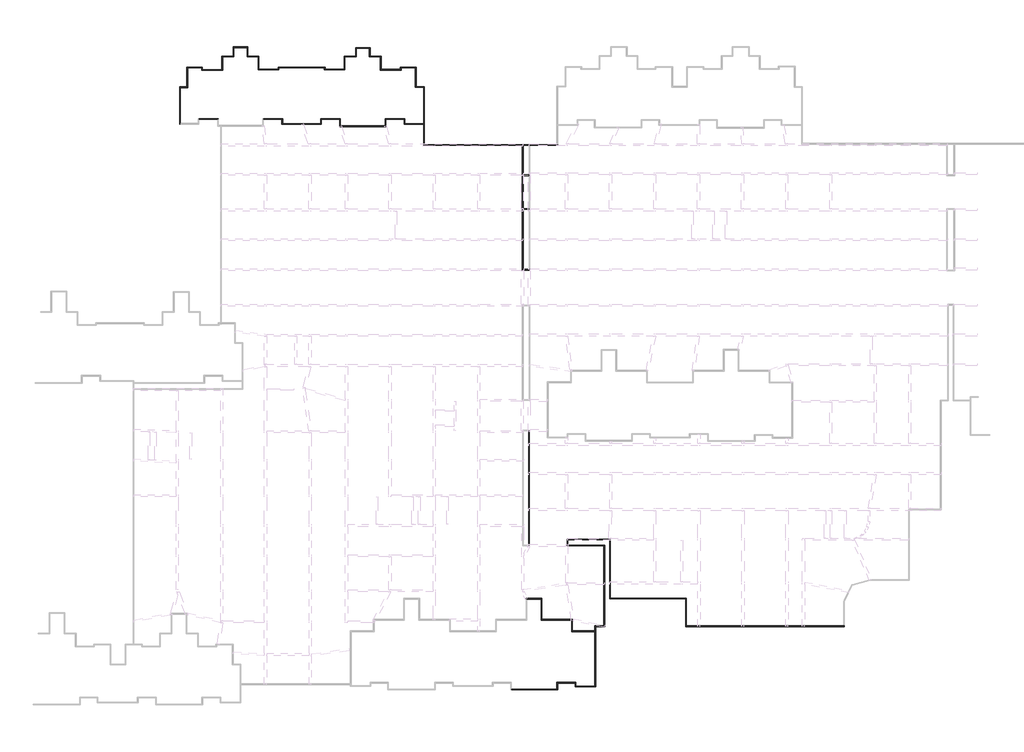
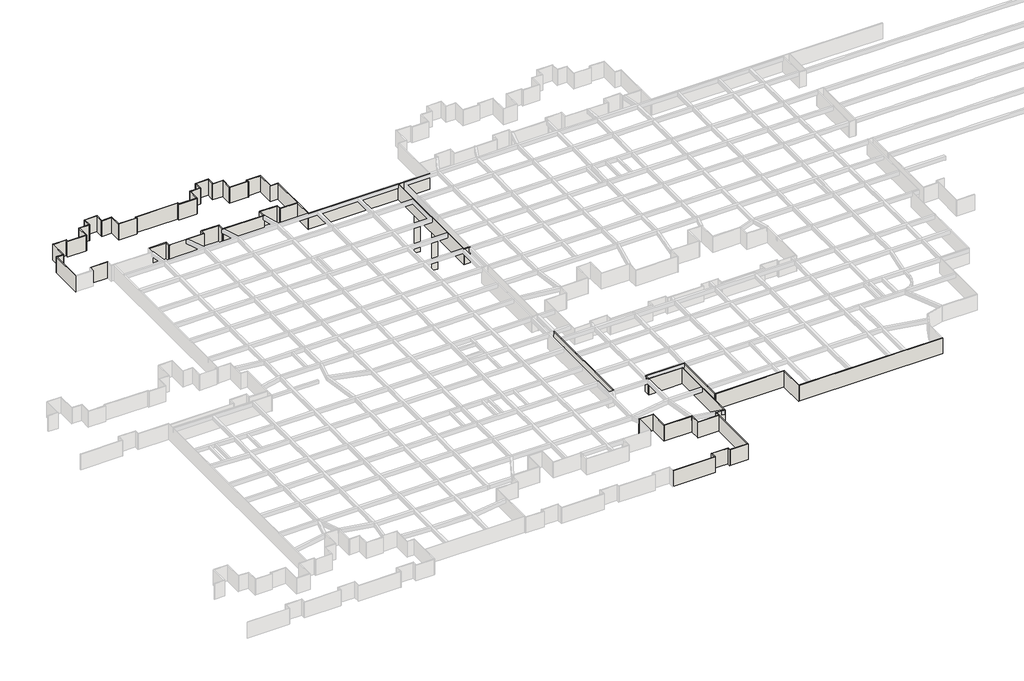
# One storey, part 3 of 16: 69 walls.
"""IFC4 building model written with IfcOpenShell, lengths in millimetres."""

from ifc_helpers import new_model, si_unit, frame, origin, origin_with_axes, place, context, project, spatial, polyline, outline, extrude, faceted_brep, element, save

model = new_model("IFC4")

# Units and contexts
model_context = context("Model", 3, world=origin())
ifc_project = project(units=[si_unit("LENGTHUNIT", "METRE", prefix="MILLI")], contexts=[model_context])

# Site, building, storey
site = spatial("IfcSite", under=ifc_project)
building = spatial("IfcBuilding", under=site)
storey = spatial("IfcBuildingStorey", under=building, Name="户型图", Elevation=0.0)

# Walls
placement = place(None, origin())
element("IfcWall", 1, ObjectType="所有墙体", at=placement, inside=storey, context=model_context, shape_type="Brep", body=[
    faceted_brep([(194060.3346415, -118367.7118415, 0.0), (194060.3346415, -121966.8447717, 0.0), (194060.3346415, -122086.8447717, 0.0), (194060.3346415, -122086.8447717, 3300.0), (194060.3346415, -121966.8447717, 3300.0), (194060.3346415, -118367.7118415, 3300.0), (194180.3346415, -118367.7118415, 0.0), (194180.3346415, -118367.7118415, 3300.0), (194180.3346415, -118487.7118415, 3300.0), (194180.3346415, -122086.8447717, 3300.0), (194180.3346415, -122086.8447717, 0.0), (194180.3346415, -118487.7118415, 0.0)], [[[0, 1, 2, 3, 4, 5]], [[6, 7, 8, 9, 10, 11]], [[2, 1, 0, 6, 11, 10]], [[5, 4, 3, 9, 8, 7]], [[3, 2, 10, 9]], [[0, 5, 7, 6]]]),
])
element("IfcWall", 2, ObjectType="所有墙体", at=placement, inside=storey, context=model_context, shape_type="Brep", body=[
    faceted_brep([(194060.3346415, -121966.8447717, 0.0), (192706.317546, -121966.8447717, 0.0), (192706.317546, -121966.8447717, 3300.0), (194060.3346415, -121966.8447717, 3300.0), (194060.3346415, -122086.8447717, 0.0), (194060.3346415, -122086.8447717, 3300.0), (192826.317546, -122086.8447717, 3300.0), (192706.317546, -122086.8447717, 3300.0), (192706.317546, -122086.8447717, 0.0), (192826.317546, -122086.8447717, 0.0)], [[[0, 1, 2, 3]], [[4, 5, 6, 7, 8, 9]], [[1, 0, 4, 9, 8]], [[3, 2, 7, 6, 5]], [[0, 3, 5, 4]], [[2, 1, 8, 7]]]),
])
element("IfcWall", 3, ObjectType="所有墙体", at=placement, inside=storey, context=model_context, shape_type="Brep", body=[
    faceted_brep([(192706.317546, -122086.8447717, 0.0), (192706.317546, -128736.151487, 0.0), (192706.317546, -128736.151487, 3300.0), (192706.317546, -122086.8447717, 3300.0), (192826.317546, -122086.8447717, 0.0), (192826.317546, -122086.8447717, 3300.0), (192826.317546, -128616.151487, 3300.0), (192826.317546, -128736.151487, 3300.0), (192826.317546, -128736.151487, 0.0), (192826.317546, -128616.151487, 0.0)], [[[0, 1, 2, 3]], [[4, 5, 6, 7, 8, 9]], [[1, 0, 4, 9, 8]], [[3, 2, 7, 6, 5]], [[0, 3, 5, 4]], [[2, 1, 8, 7]]]),
])
element("IfcWall", 4, ObjectType="所有墙体", at=placement, inside=storey, context=model_context, shape_type="Brep", body=[
    faceted_brep([(196226.317546, -127836.151487, 0.0), (199599.9062186, -127836.151487, 0.0), (199719.9062186, -127836.151487, 0.0), (199719.9062186, -127836.151487, 3300.0), (199599.9062186, -127836.151487, 3300.0), (196226.317546, -127836.151487, 3300.0), (196226.317546, -127716.151487, 0.0), (196226.317546, -127716.151487, 3300.0), (199719.9062186, -127716.151487, 3300.0), (199719.9062186, -127716.151487, 0.0)], [[[0, 1, 2, 3, 4, 5]], [[6, 7, 8, 9]], [[2, 1, 0, 6, 9]], [[5, 4, 3, 8, 7]], [[0, 5, 7, 6]], [[3, 2, 9, 8]]]),
])
element("IfcWall", 5, ObjectType="所有墙体", at=placement, inside=storey, context=model_context, shape_type="Brep", body=[
    faceted_brep([(207918.5069416, -127836.151487, 0.0), (211299.9135032, -127836.151487, 0.0), (211419.9135032, -127836.151487, 0.0), (211419.9135032, -127836.151487, 3300.0), (211299.9135032, -127836.151487, 3300.0), (207918.5069416, -127836.151487, 3300.0), (207918.5069416, -127716.151487, 0.0), (207918.5069416, -127716.151487, 3300.0), (211419.9135032, -127716.151487, 3300.0), (211419.9135032, -127716.151487, 0.0)], [[[0, 1, 2, 3, 4, 5]], [[6, 7, 8, 9]], [[2, 1, 0, 6, 9]], [[5, 4, 3, 8, 7]], [[0, 5, 7, 6]], [[3, 2, 9, 8]]]),
])
element("IfcWall", 6, ObjectType="所有墙体", at=placement, inside=storey, context=model_context, shape_type="Brep", body=[
    faceted_brep([(211299.9135032, -127836.151487, 0.0), (211299.9135032, -128756.8999905, 0.0), (211299.9135032, -128756.8999905, 3300.0), (211299.9135032, -127836.151487, 3300.0), (211419.9135032, -127836.151487, 0.0), (211419.9135032, -127836.151487, 3300.0), (211419.9135032, -128636.8999905, 3300.0), (211419.9135032, -128756.8999905, 3300.0), (211419.9135032, -128756.8999905, 0.0), (211419.9135032, -128636.8999905, 0.0)], [[[0, 1, 2, 3]], [[4, 5, 6, 7, 8, 9]], [[1, 0, 4, 9, 8]], [[3, 2, 7, 6, 5]], [[0, 3, 5, 4]], [[2, 1, 8, 7]]]),
])
element("IfcWall", 7, ObjectType="所有墙体", at=placement, inside=storey, context=model_context, shape_type="Brep", body=[
    faceted_brep([(211419.9135032, -128756.8999905, 0.0), (218418.8904026, -128756.8999905, 0.0), (218418.8904026, -128756.8999905, 3300.0), (211419.9135032, -128756.8999905, 3300.0), (211419.9135032, -128636.8999905, 0.0), (211419.9135032, -128636.8999905, 3300.0), (218298.8904026, -128636.8999905, 3300.0), (218418.8904026, -128636.8999905, 3300.0), (218418.8904026, -128636.8999905, 0.0), (218298.8904026, -128636.8999905, 0.0)], [[[0, 1, 2, 3]], [[4, 5, 6, 7, 8, 9]], [[1, 0, 4, 9, 8]], [[3, 2, 7, 6, 5]], [[0, 3, 5, 4]], [[2, 1, 8, 7]]]),
])
element("IfcWall", 8, ObjectType="所有墙体", at=placement, inside=storey, context=model_context, shape_type="Brep", body=[
    faceted_brep([(218418.8904026, -128636.8999905, 0.0), (218418.8904026, -127836.151487, 0.0), (218418.8904026, -127716.151487, 0.0), (218418.8904026, -127716.151487, 3300.0), (218418.8904026, -127836.151487, 3300.0), (218418.8904026, -128636.8999905, 3300.0), (218298.8904026, -128636.8999905, 0.0), (218298.8904026, -128636.8999905, 3300.0), (218298.8904026, -127716.151487, 3300.0), (218298.8904026, -127716.151487, 0.0)], [[[0, 1, 2, 3, 4, 5]], [[6, 7, 8, 9]], [[2, 1, 0, 6, 9]], [[5, 4, 3, 8, 7]], [[0, 5, 7, 6]], [[3, 2, 9, 8]]]),
])
element("IfcWall", 9, ObjectType="所有墙体", at=placement, inside=storey, context=model_context, shape_type="Brep", body=[
    faceted_brep([(218418.8904026, -127836.151487, 0.0), (221799.9200406, -127836.151487, 0.0), (221919.9200406, -127836.151487, 0.0), (221919.9200406, -127836.151487, 3300.0), (221799.9200406, -127836.151487, 3300.0), (218418.8904026, -127836.151487, 3300.0), (218418.8904026, -127716.151487, 0.0), (218418.8904026, -127716.151487, 3300.0), (221919.9200406, -127716.151487, 3300.0), (221919.9200406, -127716.151487, 0.0)], [[[0, 1, 2, 3, 4, 5]], [[6, 7, 8, 9]], [[2, 1, 0, 6, 9]], [[5, 4, 3, 8, 7]], [[0, 5, 7, 6]], [[3, 2, 9, 8]]]),
])
element("IfcWall", 10, ObjectType="所有墙体", at=placement, inside=storey, context=model_context, shape_type="Brep", body=[
    faceted_brep([(221799.9200406, -127836.151487, 0.0), (221799.9200406, -129168.6171458, 0.0), (221799.9200406, -129168.6171458, 3300.0), (221799.9200406, -127836.151487, 3300.0), (221919.9200406, -127836.151487, 0.0), (221919.9200406, -127836.151487, 3300.0), (221919.9200406, -129048.6171458, 3300.0), (221919.9200406, -129168.6171458, 3300.0), (221919.9200406, -129168.6171458, 0.0), (221919.9200406, -129048.6171458, 0.0)], [[[0, 1, 2, 3]], [[4, 5, 6, 7, 8, 9]], [[1, 0, 4, 9, 8]], [[3, 2, 7, 6, 5]], [[0, 3, 5, 4]], [[2, 1, 8, 7]]]),
])
element("IfcWall", 11, ObjectType="所有墙体", at=placement, inside=storey, context=model_context, shape_type="Brep", body=[
    faceted_brep([(221919.9200406, -129168.6171458, 0.0), (230118.438254, -129168.6171458, 0.0), (230118.438254, -129168.6171458, 3300.0), (221919.9200406, -129168.6171458, 3300.0), (221919.9200406, -129048.6171458, 0.0), (221919.9200406, -129048.6171458, 3300.0), (229998.438254, -129048.6171458, 3300.0), (230118.438254, -129048.6171458, 3300.0), (230118.438254, -129048.6171458, 0.0), (229998.438254, -129048.6171458, 0.0)], [[[0, 1, 2, 3]], [[4, 5, 6, 7, 8, 9]], [[1, 0, 4, 9, 8]], [[3, 2, 7, 6, 5]], [[0, 3, 5, 4]], [[2, 1, 8, 7]]]),
])
element("IfcWall", 12, ObjectType="所有墙体", at=placement, inside=storey, context=model_context, shape_type="Brep", body=[
    faceted_brep([(230118.438254, -129048.6171458, 0.0), (230118.438254, -127836.151487, 0.0), (230118.438254, -127716.151487, 0.0), (230118.438254, -127716.151487, 3300.0), (230118.438254, -127836.151487, 3300.0), (230118.438254, -129048.6171458, 3300.0), (229998.438254, -129048.6171458, 0.0), (229998.438254, -129048.6171458, 3300.0), (229998.438254, -127716.151487, 3300.0), (229998.438254, -127716.151487, 0.0)], [[[0, 1, 2, 3, 4, 5]], [[6, 7, 8, 9]], [[2, 1, 0, 6, 9]], [[5, 4, 3, 8, 7]], [[0, 5, 7, 6]], [[3, 2, 9, 8]]]),
])
element("IfcWall", 13, ObjectType="所有墙体", at=placement, inside=storey, context=model_context, shape_type="Brep", body=[
    faceted_brep([(230118.438254, -127836.151487, 0.0), (233499.9273251, -127836.151487, 0.0), (233619.9273251, -127836.151487, 0.0), (233619.9273251, -127836.151487, 3300.0), (233499.9273251, -127836.151487, 3300.0), (230118.438254, -127836.151487, 3300.0), (230118.438254, -127716.151487, 0.0), (230118.438254, -127716.151487, 3300.0), (233619.9273251, -127716.151487, 3300.0), (233619.9273251, -127716.151487, 0.0)], [[[0, 1, 2, 3, 4, 5]], [[6, 7, 8, 9]], [[2, 1, 0, 6, 9]], [[5, 4, 3, 8, 7]], [[0, 5, 7, 6]], [[3, 2, 9, 8]]]),
])
element("IfcWall", 14, ObjectType="所有墙体", at=placement, inside=storey, context=model_context, shape_type="Brep", body=[
    faceted_brep([(233499.9273251, -127836.151487, 0.0), (233499.9273251, -128756.8999905, 0.0), (233499.9273251, -128756.8999905, 3300.0), (233499.9273251, -127836.151487, 3300.0), (233619.9273251, -127836.151487, 0.0), (233619.9273251, -127836.151487, 3300.0), (233619.9273251, -128636.8999905, 3300.0), (233619.9273251, -128756.8999905, 3300.0), (233619.9273251, -128756.8999905, 0.0), (233619.9273251, -128636.8999905, 0.0)], [[[0, 1, 2, 3]], [[4, 5, 6, 7, 8, 9]], [[1, 0, 4, 9, 8]], [[3, 2, 7, 6, 5]], [[0, 3, 5, 4]], [[2, 1, 8, 7]]]),
])
element("IfcWall", 15, ObjectType="所有墙体", at=placement, inside=storey, context=model_context, shape_type="SweptSolid", body=[
    extrude(outline(polyline([(237002.7517568, -128756.8999905), (233619.9273251, -128756.8999905), (233619.9273251, -128636.8999905), (237002.7517568, -128636.8999905), (237002.7517568, -128756.8999905)])), origin_with_axes(), (0.0, 0.0, 1.0), 3300.0),
])
element("IfcWall", 16, ObjectType="所有墙体", at=placement, inside=storey, context=model_context, shape_type="Brep", body=[
    faceted_brep([(237122.7517568, -132556.8999905, 0.0), (237122.7517568, -132436.8999905, 0.0), (237122.7517568, -121914.0192789, 0.0), (237122.7517568, -121914.0192789, 3300.0), (237122.7517568, -132436.8999905, 3300.0), (237122.7517568, -132556.8999905, 3300.0), (237002.7517568, -132556.8999905, 0.0), (237002.7517568, -132556.8999905, 3300.0), (237002.7517568, -128756.8999905, 3300.0), (237002.7517568, -128636.8999905, 3300.0), (237002.7517568, -122034.0192789, 3300.0), (237002.7517568, -121914.0192789, 3300.0), (237002.7517568, -121914.0192789, 0.0), (237002.7517568, -122034.0192789, 0.0), (237002.7517568, -128636.8999905, 0.0), (237002.7517568, -128756.8999905, 0.0)], [[[0, 1, 2, 3, 4, 5]], [[6, 7, 8, 9, 10, 11, 12, 13, 14, 15]], [[2, 1, 0, 6, 15, 14, 13, 12]], [[5, 4, 3, 11, 10, 9, 8, 7]], [[3, 2, 12, 11]], [[0, 5, 7, 6]]]),
])
element("IfcWall", 17, ObjectType="所有墙体", at=placement, inside=storey, context=model_context, shape_type="Brep", body=[
    faceted_brep([(237002.7517568, -121914.0192789, 0.0), (235628.9140291, -121914.0192789, 0.0), (235508.9140291, -121914.0192789, 0.0), (235508.9140291, -121914.0192789, 3300.0), (235628.9140291, -121914.0192789, 3300.0), (237002.7517568, -121914.0192789, 3300.0), (237002.7517568, -122034.0192789, 0.0), (237002.7517568, -122034.0192789, 3300.0), (235508.9140291, -122034.0192789, 3300.0), (235508.9140291, -122034.0192789, 0.0)], [[[0, 1, 2, 3, 4, 5]], [[6, 7, 8, 9]], [[2, 1, 0, 6, 9]], [[5, 4, 3, 8, 7]], [[0, 5, 7, 6]], [[3, 2, 9, 8]]]),
])
element("IfcWall", 18, ObjectType="所有墙体", at=placement, inside=storey, context=model_context, shape_type="Brep", body=[
    faceted_brep([(235628.9140291, -121914.0192789, 0.0), (235628.9140291, -118412.2081323, 0.0), (235628.9140291, -118412.2081323, 3300.0), (235628.9140291, -121914.0192789, 3300.0), (235508.9140291, -121914.0192789, 0.0), (235508.9140291, -121914.0192789, 3300.0), (235508.9140291, -118532.2081323, 3300.0), (235508.9140291, -118412.2081323, 3300.0), (235508.9140291, -118412.2081323, 0.0), (235508.9140291, -118532.2081323, 0.0)], [[[0, 1, 2, 3]], [[4, 5, 6, 7, 8, 9]], [[1, 0, 4, 9, 8]], [[3, 2, 7, 6, 5]], [[0, 3, 5, 4]], [[2, 1, 8, 7]]]),
])
element("IfcWall", 19, ObjectType="所有墙体", at=placement, inside=storey, context=model_context, shape_type="Brep", body=[
    faceted_brep([(235508.9140291, -118412.2081323, 0.0), (232809.8642198, -118412.2081323, 0.0), (232809.8642198, -118412.2081323, 3300.0), (235508.9140291, -118412.2081323, 3300.0), (235508.9140291, -118532.2081323, 0.0), (235508.9140291, -118532.2081323, 3300.0), (232929.8642198, -118532.2081323, 3300.0), (232809.8642198, -118532.2081323, 3300.0), (232809.8642198, -118532.2081323, 0.0), (232929.8642198, -118532.2081323, 0.0)], [[[0, 1, 2, 3]], [[4, 5, 6, 7, 8, 9]], [[1, 0, 4, 9, 8]], [[3, 2, 7, 6, 5]], [[0, 3, 5, 4]], [[2, 1, 8, 7]]]),
])
element("IfcWall", 20, ObjectType="所有墙体", at=placement, inside=storey, context=model_context, shape_type="Brep", body=[
    faceted_brep([(232809.8642198, -118532.2081323, 0.0), (232809.8642198, -118808.218552, 0.0), (232809.8642198, -118928.218552, 0.0), (232809.8642198, -118928.218552, 3300.0), (232809.8642198, -118808.218552, 3300.0), (232809.8642198, -118532.2081323, 3300.0), (232929.8642198, -118532.2081323, 0.0), (232929.8642198, -118532.2081323, 3300.0), (232929.8642198, -118928.218552, 3300.0), (232929.8642198, -118928.218552, 0.0)], [[[0, 1, 2, 3, 4, 5]], [[6, 7, 8, 9]], [[2, 1, 0, 6, 9]], [[5, 4, 3, 8, 7]], [[0, 5, 7, 6]], [[3, 2, 9, 8]]]),
])
element("IfcWall", 21, ObjectType="所有墙体", at=placement, inside=storey, context=model_context, shape_type="Brep", body=[
    faceted_brep([(232809.8642198, -118808.218552, 0.0), (229282.488847, -118808.218552, 0.0), (229162.488847, -118808.218552, 0.0), (229162.488847, -118808.218552, 3300.0), (229282.488847, -118808.218552, 3300.0), (232809.8642198, -118808.218552, 3300.0), (232809.8642198, -118928.218552, 0.0), (232809.8642198, -118928.218552, 3300.0), (229162.488847, -118928.218552, 3300.0), (229162.488847, -118928.218552, 0.0)], [[[0, 1, 2, 3, 4, 5]], [[6, 7, 8, 9]], [[2, 1, 0, 6, 9]], [[5, 4, 3, 8, 7]], [[0, 5, 7, 6]], [[3, 2, 9, 8]]]),
])
element("IfcWall", 22, ObjectType="所有墙体", at=placement, inside=storey, context=model_context, shape_type="Brep", body=[
    faceted_brep([(229282.488847, -118808.218552, 0.0), (229282.488847, -116405.5418968, 0.0), (229282.488847, -116405.5418968, 3300.0), (229282.488847, -118808.218552, 3300.0), (229162.488847, -118808.218552, 0.0), (229162.488847, -118808.218552, 3300.0), (229162.488847, -116525.5418968, 3300.0), (229162.488847, -116405.5418968, 3300.0), (229162.488847, -116405.5418968, 0.0), (229162.488847, -116525.5418968, 0.0)], [[[0, 1, 2, 3]], [[4, 5, 6, 7, 8, 9]], [[1, 0, 4, 9, 8]], [[3, 2, 7, 6, 5]], [[0, 3, 5, 4]], [[2, 1, 8, 7]]]),
])
element("IfcWall", 23, ObjectType="所有墙体", at=placement, inside=storey, context=model_context, shape_type="Brep", body=[
    faceted_brep([(229162.488847, -116405.5418968, 0.0), (227283.5491439, -116405.5418968, 0.0), (227163.5491439, -116405.5418968, 0.0), (227163.5491439, -116405.5418968, 3300.0), (227283.5491439, -116405.5418968, 3300.0), (229162.488847, -116405.5418968, 3300.0), (229162.488847, -116525.5418968, 0.0), (229162.488847, -116525.5418968, 3300.0), (227163.5491439, -116525.5418968, 3300.0), (227163.5491439, -116525.5418968, 0.0)], [[[0, 1, 2, 3, 4, 5]], [[6, 7, 8, 9]], [[2, 1, 0, 6, 9]], [[5, 4, 3, 8, 7]], [[0, 5, 7, 6]], [[3, 2, 9, 8]]]),
])
element("IfcWall", 24, ObjectType="所有墙体", at=placement, inside=storey, context=model_context, shape_type="Brep", body=[
    faceted_brep([(227283.5491439, -116405.5418968, 0.0), (227283.5491439, -114851.8046012, 0.0), (227283.5491439, -114851.8046012, 3300.0), (227283.5491439, -116405.5418968, 3300.0), (227163.5491439, -116405.5418968, 0.0), (227163.5491439, -116405.5418968, 3300.0), (227163.5491439, -114971.8046012, 3300.0), (227163.5491439, -114851.8046012, 3300.0), (227163.5491439, -114851.8046012, 0.0), (227163.5491439, -114971.8046012, 0.0)], [[[0, 1, 2, 3]], [[4, 5, 6, 7, 8, 9]], [[1, 0, 4, 9, 8]], [[3, 2, 7, 6, 5]], [[0, 3, 5, 4]], [[2, 1, 8, 7]]]),
])
element("IfcWall", 25, ObjectType="所有墙体", at=placement, inside=storey, context=model_context, shape_type="Brep", body=[
    faceted_brep([(227163.5491439, -114851.8046012, 0.0), (224663.3843746, -114851.8046012, 0.0), (224663.3843746, -114851.8046012, 3300.0), (227163.5491439, -114851.8046012, 3300.0), (227163.5491439, -114971.8046012, 0.0), (227163.5491439, -114971.8046012, 3300.0), (224783.3843746, -114971.8046012, 3300.0), (224663.3843746, -114971.8046012, 3300.0), (224663.3843746, -114971.8046012, 0.0), (224783.3843746, -114971.8046012, 0.0)], [[[0, 1, 2, 3]], [[4, 5, 6, 7, 8, 9]], [[1, 0, 4, 9, 8]], [[3, 2, 7, 6, 5]], [[0, 3, 5, 4]], [[2, 1, 8, 7]]]),
])
element("IfcWall", 26, ObjectType="所有墙体", at=placement, inside=storey, context=model_context, shape_type="Brep", body=[
    faceted_brep([(224663.3843746, -114971.8046012, 0.0), (224663.3843746, -116405.5418968, 0.0), (224663.3843746, -116525.5418968, 0.0), (224663.3843746, -116525.5418968, 3300.0), (224663.3843746, -116405.5418968, 3300.0), (224663.3843746, -114971.8046012, 3300.0), (224783.3843746, -114971.8046012, 0.0), (224783.3843746, -114971.8046012, 3300.0), (224783.3843746, -116525.5418968, 3300.0), (224783.3843746, -116525.5418968, 0.0)], [[[0, 1, 2, 3, 4, 5]], [[6, 7, 8, 9]], [[2, 1, 0, 6, 9]], [[5, 4, 3, 8, 7]], [[0, 5, 7, 6]], [[3, 2, 9, 8]]]),
])
element("IfcWall", 27, ObjectType="所有墙体", at=placement, inside=storey, context=model_context, shape_type="Brep", body=[
    faceted_brep([(224663.3843746, -116405.5418968, 0.0), (222610.0704279, -116405.5418968, 0.0), (222610.0704279, -116405.5418968, 3300.0), (224663.3843746, -116405.5418968, 3300.0), (224663.3843746, -116525.5418968, 0.0), (224663.3843746, -116525.5418968, 3300.0), (222730.0704279, -116525.5418968, 3300.0), (222610.0704279, -116525.5418968, 3300.0), (222610.0704279, -116525.5418968, 0.0), (222730.0704279, -116525.5418968, 0.0)], [[[0, 1, 2, 3]], [[4, 5, 6, 7, 8, 9]], [[1, 0, 4, 9, 8]], [[3, 2, 7, 6, 5]], [[0, 3, 5, 4]], [[2, 1, 8, 7]]]),
])
element("IfcWall", 28, ObjectType="所有墙体", at=placement, inside=storey, context=model_context, shape_type="Brep", body=[
    faceted_brep([(222610.0704279, -116525.5418968, 0.0), (222610.0704279, -118749.3864331, 0.0), (222610.0704279, -118869.3864331, 0.0), (222610.0704279, -118869.3864331, 3300.0), (222610.0704279, -118749.3864331, 3300.0), (222610.0704279, -116525.5418968, 3300.0), (222730.0704279, -116525.5418968, 0.0), (222730.0704279, -116525.5418968, 3300.0), (222730.0704279, -118869.3864331, 3300.0), (222730.0704279, -118869.3864331, 0.0)], [[[0, 1, 2, 3, 4, 5]], [[6, 7, 8, 9]], [[2, 1, 0, 6, 9]], [[5, 4, 3, 8, 7]], [[0, 5, 7, 6]], [[3, 2, 9, 8]]]),
])
element("IfcWall", 29, ObjectType="所有墙体", at=placement, inside=storey, context=model_context, shape_type="Brep", body=[
    faceted_brep([(222610.0704279, -118749.3864331, 0.0), (219130.3191805, -118749.3864331, 0.0), (219010.3191805, -118749.3864331, 0.0), (219010.3191805, -118749.3864331, 3300.0), (219130.3191805, -118749.3864331, 3300.0), (222610.0704279, -118749.3864331, 3300.0), (222610.0704279, -118869.3864331, 0.0), (222610.0704279, -118869.3864331, 3300.0), (219010.3191805, -118869.3864331, 3300.0), (219010.3191805, -118869.3864331, 0.0)], [[[0, 1, 2, 3, 4, 5]], [[6, 7, 8, 9]], [[2, 1, 0, 6, 9]], [[5, 4, 3, 8, 7]], [[0, 5, 7, 6]], [[3, 2, 9, 8]]]),
])
element("IfcWall", 30, ObjectType="所有墙体", at=placement, inside=storey, context=model_context, shape_type="Brep", body=[
    faceted_brep([(219130.3191805, -118749.3864331, 0.0), (219130.3191805, -118390.5039842, 0.0), (219130.3191805, -118390.5039842, 3300.0), (219130.3191805, -118749.3864331, 3300.0), (219010.3191805, -118749.3864331, 0.0), (219010.3191805, -118749.3864331, 3300.0), (219010.3191805, -118510.5039842, 3300.0), (219010.3191805, -118390.5039842, 3300.0), (219010.3191805, -118390.5039842, 0.0), (219010.3191805, -118510.5039842, 0.0)], [[[0, 1, 2, 3]], [[4, 5, 6, 7, 8, 9]], [[1, 0, 4, 9, 8]], [[3, 2, 7, 6, 5]], [[0, 3, 5, 4]], [[2, 1, 8, 7]]]),
])
element("IfcWall", 31, ObjectType="所有墙体", at=placement, inside=storey, context=model_context, shape_type="Brep", body=[
    faceted_brep([(219010.3191805, -118390.5039842, 0.0), (210609.9338471, -118390.5039842, 0.0), (210609.9338471, -118390.5039842, 3300.0), (219010.3191805, -118390.5039842, 3300.0), (219010.3191805, -118510.5039842, 0.0), (219010.3191805, -118510.5039842, 3300.0), (210729.9338471, -118510.5039842, 3300.0), (210609.9338471, -118510.5039842, 3300.0), (210609.9338471, -118510.5039842, 0.0), (210729.9338471, -118510.5039842, 0.0)], [[[0, 1, 2, 3]], [[4, 5, 6, 7, 8, 9]], [[1, 0, 4, 9, 8]], [[3, 2, 7, 6, 5]], [[0, 3, 5, 4]], [[2, 1, 8, 7]]]),
])
element("IfcWall", 32, ObjectType="所有墙体", at=placement, inside=storey, context=model_context, shape_type="Brep", body=[
    faceted_brep([(210609.9338471, -118510.5039842, 0.0), (210609.9338471, -118749.3864331, 0.0), (210609.9338471, -118869.3864331, 0.0), (210609.9338471, -118869.3864331, 3300.0), (210609.9338471, -118749.3864331, 3300.0), (210609.9338471, -118510.5039842, 3300.0), (210729.9338471, -118510.5039842, 0.0), (210729.9338471, -118510.5039842, 3300.0), (210729.9338471, -118869.3864331, 3300.0), (210729.9338471, -118869.3864331, 0.0)], [[[0, 1, 2, 3, 4, 5]], [[6, 7, 8, 9]], [[2, 1, 0, 6, 9]], [[5, 4, 3, 8, 7]], [[0, 5, 7, 6]], [[3, 2, 9, 8]]]),
])
element("IfcWall", 33, ObjectType="所有墙体", at=placement, inside=storey, context=model_context, shape_type="Brep", body=[
    faceted_brep([(210609.9338471, -118749.3864331, 0.0), (207082.5026691, -118749.3864331, 0.0), (206962.5026691, -118749.3864331, 0.0), (206962.5026691, -118749.3864331, 3300.0), (207082.5026691, -118749.3864331, 3300.0), (210609.9338471, -118749.3864331, 3300.0), (210609.9338471, -118869.3864331, 0.0), (210609.9338471, -118869.3864331, 3300.0), (206962.5026691, -118869.3864331, 3300.0), (206962.5026691, -118869.3864331, 0.0)], [[[0, 1, 2, 3, 4, 5]], [[6, 7, 8, 9]], [[2, 1, 0, 6, 9]], [[5, 4, 3, 8, 7]], [[0, 5, 7, 6]], [[3, 2, 9, 8]]]),
])
element("IfcWall", 34, ObjectType="所有墙体", at=placement, inside=storey, context=model_context, shape_type="Brep", body=[
    faceted_brep([(207082.5026691, -118749.3864331, 0.0), (207082.5026691, -116405.5418968, 0.0), (207082.5026691, -116405.5418968, 3300.0), (207082.5026691, -118749.3864331, 3300.0), (206962.5026691, -118749.3864331, 0.0), (206962.5026691, -118749.3864331, 3300.0), (206962.5026691, -116525.5418968, 3300.0), (206962.5026691, -116405.5418968, 3300.0), (206962.5026691, -116405.5418968, 0.0), (206962.5026691, -116525.5418968, 0.0)], [[[0, 1, 2, 3]], [[4, 5, 6, 7, 8, 9]], [[1, 0, 4, 9, 8]], [[3, 2, 7, 6, 5]], [[0, 3, 5, 4]], [[2, 1, 8, 7]]]),
])
element("IfcWall", 35, ObjectType="所有墙体", at=placement, inside=storey, context=model_context, shape_type="Brep", body=[
    faceted_brep([(206962.5026691, -116405.5418968, 0.0), (205085.2649614, -116405.5418968, 0.0), (204965.2649614, -116405.5418968, 0.0), (204965.2649614, -116405.5418968, 3300.0), (205085.2649614, -116405.5418968, 3300.0), (206962.5026691, -116405.5418968, 3300.0), (206962.5026691, -116525.5418968, 0.0), (206962.5026691, -116525.5418968, 3300.0), (204965.2649614, -116525.5418968, 3300.0), (204965.2649614, -116525.5418968, 0.0)], [[[0, 1, 2, 3, 4, 5]], [[6, 7, 8, 9]], [[2, 1, 0, 6, 9]], [[5, 4, 3, 8, 7]], [[0, 5, 7, 6]], [[3, 2, 9, 8]]]),
])
element("IfcWall", 36, ObjectType="所有墙体", at=placement, inside=storey, context=model_context, shape_type="Brep", body=[
    faceted_brep([(205085.2649614, -116405.5418968, 0.0), (205085.2649614, -114728.4266647, 0.0), (205085.2649614, -114728.4266647, 3300.0), (205085.2649614, -116405.5418968, 3300.0), (204965.2649614, -116405.5418968, 0.0), (204965.2649614, -116405.5418968, 3300.0), (204965.2649614, -114848.4266647, 3300.0), (204965.2649614, -114728.4266647, 3300.0), (204965.2649614, -114728.4266647, 0.0), (204965.2649614, -114848.4266647, 0.0)], [[[0, 1, 2, 3]], [[4, 5, 6, 7, 8, 9]], [[1, 0, 4, 9, 8]], [[3, 2, 7, 6, 5]], [[0, 3, 5, 4]], [[2, 1, 8, 7]]]),
])
element("IfcWall", 37, ObjectType="所有墙体", at=placement, inside=storey, context=model_context, shape_type="Brep", body=[
    faceted_brep([(204965.2649614, -114728.4266647, 0.0), (202463.5082295, -114728.4266647, 0.0), (202463.5082295, -114728.4266647, 3300.0), (204965.2649614, -114728.4266647, 3300.0), (204965.2649614, -114848.4266647, 0.0), (204965.2649614, -114848.4266647, 3300.0), (202583.5082295, -114848.4266647, 3300.0), (202463.5082295, -114848.4266647, 3300.0), (202463.5082295, -114848.4266647, 0.0), (202583.5082295, -114848.4266647, 0.0)], [[[0, 1, 2, 3]], [[4, 5, 6, 7, 8, 9]], [[1, 0, 4, 9, 8]], [[3, 2, 7, 6, 5]], [[0, 3, 5, 4]], [[2, 1, 8, 7]]]),
])
element("IfcWall", 38, ObjectType="所有墙体", at=placement, inside=storey, context=model_context, shape_type="Brep", body=[
    faceted_brep([(202463.5082295, -114848.4266647, 0.0), (202463.5082295, -116405.5418968, 0.0), (202463.5082295, -116525.5418968, 0.0), (202463.5082295, -116525.5418968, 3300.0), (202463.5082295, -116405.5418968, 3300.0), (202463.5082295, -114848.4266647, 3300.0), (202583.5082295, -114848.4266647, 0.0), (202583.5082295, -114848.4266647, 3300.0), (202583.5082295, -116525.5418968, 3300.0), (202583.5082295, -116525.5418968, 0.0)], [[[0, 1, 2, 3, 4, 5]], [[6, 7, 8, 9]], [[2, 1, 0, 6, 9]], [[5, 4, 3, 8, 7]], [[0, 5, 7, 6]], [[3, 2, 9, 8]]]),
])
element("IfcWall", 39, ObjectType="所有墙体", at=placement, inside=storey, context=model_context, shape_type="Brep", body=[
    faceted_brep([(202463.5082295, -116405.5418968, 0.0), (200410.4144423, -116405.5418968, 0.0), (200410.4144423, -116405.5418968, 3300.0), (202463.5082295, -116405.5418968, 3300.0), (202463.5082295, -116525.5418968, 0.0), (202463.5082295, -116525.5418968, 3300.0), (200530.4144423, -116525.5418968, 3300.0), (200410.4144423, -116525.5418968, 3300.0), (200410.4144423, -116525.5418968, 0.0), (200530.4144423, -116525.5418968, 0.0)], [[[0, 1, 2, 3]], [[4, 5, 6, 7, 8, 9]], [[1, 0, 4, 9, 8]], [[3, 2, 7, 6, 5]], [[0, 3, 5, 4]], [[2, 1, 8, 7]]]),
])
element("IfcWall", 40, ObjectType="所有墙体", at=placement, inside=storey, context=model_context, shape_type="Brep", body=[
    faceted_brep([(200410.4144423, -116525.5418968, 0.0), (200410.4144423, -118820.6686813, 0.0), (200410.4144423, -118940.6686813, 0.0), (200410.4144423, -118940.6686813, 3300.0), (200410.4144423, -118820.6686813, 3300.0), (200410.4144423, -116525.5418968, 3300.0), (200530.4144423, -116525.5418968, 0.0), (200530.4144423, -116525.5418968, 3300.0), (200530.4144423, -118940.6686813, 3300.0), (200530.4144423, -118940.6686813, 0.0)], [[[0, 1, 2, 3, 4, 5]], [[6, 7, 8, 9]], [[2, 1, 0, 6, 9]], [[5, 4, 3, 8, 7]], [[0, 5, 7, 6]], [[3, 2, 9, 8]]]),
])
element("IfcWall", 41, ObjectType="所有墙体", at=placement, inside=storey, context=model_context, shape_type="Brep", body=[
    faceted_brep([(200410.4144423, -118820.6686813, 0.0), (196830.4144423, -118820.6686813, 0.0), (196710.4144423, -118820.6686813, 0.0), (196710.4144423, -118820.6686813, 3300.0), (196830.4144423, -118820.6686813, 3300.0), (200410.4144423, -118820.6686813, 3300.0), (200410.4144423, -118940.6686813, 0.0), (200410.4144423, -118940.6686813, 3300.0), (196710.4144423, -118940.6686813, 3300.0), (196710.4144423, -118940.6686813, 0.0)], [[[0, 1, 2, 3, 4, 5]], [[6, 7, 8, 9]], [[2, 1, 0, 6, 9]], [[5, 4, 3, 8, 7]], [[0, 5, 7, 6]], [[3, 2, 9, 8]]]),
])
element("IfcWall", 42, ObjectType="所有墙体", at=placement, inside=storey, context=model_context, shape_type="Brep", body=[
    faceted_brep([(196830.4144423, -118820.6686813, 0.0), (196830.4144423, -118367.7118415, 0.0), (196830.4144423, -118367.7118415, 3300.0), (196830.4144423, -118820.6686813, 3300.0), (196710.4144423, -118820.6686813, 0.0), (196710.4144423, -118820.6686813, 3300.0), (196710.4144423, -118487.7118415, 3300.0), (196710.4144423, -118367.7118415, 3300.0), (196710.4144423, -118367.7118415, 0.0), (196710.4144423, -118487.7118415, 0.0)], [[[0, 1, 2, 3]], [[4, 5, 6, 7, 8, 9]], [[1, 0, 4, 9, 8]], [[3, 2, 7, 6, 5]], [[0, 3, 5, 4]], [[2, 1, 8, 7]]]),
])
element("IfcWall", 43, ObjectType="所有墙体", at=placement, inside=storey, context=model_context, shape_type="SweptSolid", body=[
    extrude(outline(polyline([(194180.3346415, -118367.7118415), (196710.4144423, -118367.7118415), (196710.4144423, -118487.7118415), (194180.3346415, -118487.7118415), (194180.3346415, -118367.7118415)])), origin_with_axes(), (0.0, 0.0, 1.0), 3300.0),
])
element("IfcWall", 44, ObjectType="所有墙体", at=placement, inside=storey, context=model_context, shape_type="Brep", body=[
    faceted_brep([(237122.7517568, -132556.8999905, 0.0), (254943.757676, -132556.8999905, 0.0), (255063.757676, -132556.8999905, 0.0), (256143.757676, -132556.8999905, 0.0), (256263.757676, -132556.8999905, 0.0), (261322.7517568, -132556.8999905, 0.0), (261322.7517568, -132556.8999905, 3300.0), (256263.757676, -132556.8999905, 3300.0), (256143.757676, -132556.8999905, 3300.0), (255063.757676, -132556.8999905, 3300.0), (254943.757676, -132556.8999905, 3300.0), (237122.7517568, -132556.8999905, 3300.0), (237122.7517568, -132436.8999905, 0.0), (237122.7517568, -132436.8999905, 3300.0), (261202.7517568, -132436.8999905, 3300.0), (261322.7517568, -132436.8999905, 3300.0), (261322.7517568, -132436.8999905, 0.0), (261202.7517568, -132436.8999905, 0.0)], [[[0, 1, 2, 3, 4, 5, 6, 7, 8, 9, 10, 11]], [[12, 13, 14, 15, 16, 17]], [[5, 4, 3, 2, 1, 0, 12, 17, 16]], [[11, 10, 9, 8, 7, 6, 15, 14, 13]], [[0, 11, 13, 12]], [[6, 5, 16, 15]]]),
])
element("IfcWall", 45, ObjectType="所有墙体", at=placement, inside=storey, context=model_context, shape_type="Brep", body=[
    faceted_brep([(252917.4720082, -231395.926057, 0.0), (261315.9847985, -231395.926057, 0.0), (261315.9847985, -231395.926057, 3300.0), (252917.4720082, -231395.926057, 3300.0), (252917.4720082, -231275.926057, 0.0), (252917.4720082, -231275.926057, 3300.0), (261195.9847985, -231275.926057, 3300.0), (261315.9847985, -231275.926057, 3300.0), (261315.9847985, -231275.926057, 0.0), (261195.9847985, -231275.926057, 0.0)], [[[0, 1, 2, 3]], [[4, 5, 6, 7, 8, 9]], [[1, 0, 4, 9, 8]], [[3, 2, 7, 6, 5]], [[0, 3, 5, 4]], [[2, 1, 8, 7]]]),
])
element("IfcWall", 46, ObjectType="所有墙体", at=placement, inside=storey, context=model_context, shape_type="Brep", body=[
    faceted_brep([(261315.9847985, -231275.926057, 0.0), (261315.9847985, -230192.9670343, 0.0), (261315.9847985, -230072.9670343, 0.0), (261315.9847985, -230072.9670343, 3300.0), (261315.9847985, -230192.9670343, 3300.0), (261315.9847985, -231275.926057, 3300.0), (261195.9847985, -231275.926057, 0.0), (261195.9847985, -231275.926057, 3300.0), (261195.9847985, -230072.9670343, 3300.0), (261195.9847985, -230072.9670343, 0.0)], [[[0, 1, 2, 3, 4, 5]], [[6, 7, 8, 9]], [[2, 1, 0, 6, 9]], [[5, 4, 3, 8, 7]], [[0, 5, 7, 6]], [[3, 2, 9, 8]]]),
])
element("IfcWall", 47, ObjectType="所有墙体", at=placement, inside=storey, context=model_context, shape_type="Brep", body=[
    faceted_brep([(261315.9847985, -230192.9670343, 0.0), (264497.4792928, -230192.9670343, 0.0), (264617.4792928, -230192.9670343, 0.0), (264617.4792928, -230192.9670343, 3300.0), (264497.4792928, -230192.9670343, 3300.0), (261315.9847985, -230192.9670343, 3300.0), (261315.9847985, -230072.9670343, 0.0), (261315.9847985, -230072.9670343, 3300.0), (264617.4792928, -230072.9670343, 3300.0), (264617.4792928, -230072.9670343, 0.0)], [[[0, 1, 2, 3, 4, 5]], [[6, 7, 8, 9]], [[2, 1, 0, 6, 9]], [[5, 4, 3, 8, 7]], [[0, 5, 7, 6]], [[3, 2, 9, 8]]]),
])
element("IfcWall", 48, ObjectType="所有墙体", at=placement, inside=storey, context=model_context, shape_type="Brep", body=[
    faceted_brep([(264497.4792928, -230192.9670343, 0.0), (264497.4792928, -230833.7545432, 0.0), (264497.4792928, -230833.7545432, 3300.0), (264497.4792928, -230192.9670343, 3300.0), (264617.4792928, -230192.9670343, 0.0), (264617.4792928, -230192.9670343, 3300.0), (264617.4792928, -230713.7545432, 3300.0), (264617.4792928, -230833.7545432, 3300.0), (264617.4792928, -230833.7545432, 0.0), (264617.4792928, -230713.7545432, 0.0)], [[[0, 1, 2, 3]], [[4, 5, 6, 7, 8, 9]], [[1, 0, 4, 9, 8]], [[3, 2, 7, 6, 5]], [[0, 3, 5, 4]], [[2, 1, 8, 7]]]),
])
element("IfcWall", 49, ObjectType="所有墙体", at=placement, inside=storey, context=model_context, shape_type="Brep", body=[
    faceted_brep([(264617.4792928, -230833.7545432, 0.0), (268216.8453205, -230833.7545432, 0.0), (268216.8453205, -230833.7545432, 3300.0), (264617.4792928, -230833.7545432, 3300.0), (264617.4792928, -230713.7545432, 0.0), (264617.4792928, -230713.7545432, 3300.0), (268096.8453205, -230713.7545432, 3300.0), (268216.8453205, -230713.7545432, 3300.0), (268216.8453205, -230713.7545432, 0.0), (268096.8453205, -230713.7545432, 0.0)], [[[0, 1, 2, 3]], [[4, 5, 6, 7, 8, 9]], [[1, 0, 4, 9, 8]], [[3, 2, 7, 6, 5]], [[0, 3, 5, 4]], [[2, 1, 8, 7]]]),
])
element("IfcWall", 50, ObjectType="所有墙体", at=placement, inside=storey, context=model_context, shape_type="Brep", body=[
    faceted_brep([(268216.8453205, -230713.7545432, 0.0), (268216.8453205, -219933.7545432, 0.0), (268216.8453205, -219813.7545432, 0.0), (268216.8453205, -219813.7545432, 3300.0), (268216.8453205, -219933.7545432, 3300.0), (268216.8453205, -230713.7545432, 3300.0), (268096.8453205, -230713.7545432, 0.0), (268096.8453205, -230713.7545432, 3300.0), (268096.8453205, -220833.7545432, 3300.0), (268096.8453205, -220713.7545432, 3300.0), (268096.8453205, -219813.7545432, 3300.0), (268096.8453205, -219813.7545432, 0.0), (268096.8453205, -220713.7545432, 0.0), (268096.8453205, -220833.7545432, 0.0)], [[[0, 1, 2, 3, 4, 5]], [[6, 7, 8, 9, 10, 11, 12, 13]], [[2, 1, 0, 6, 13, 12, 11]], [[5, 4, 3, 10, 9, 8, 7]], [[0, 5, 7, 6]], [[3, 2, 11, 10]]]),
])
element("IfcWall", 51, ObjectType="所有墙体", at=placement, inside=storey, context=model_context, shape_type="Brep", body=[
    faceted_brep([(268096.8453205, -220713.7545432, 0.0), (264027.0023283, -220713.7545432, 0.0), (263907.0023283, -220713.7545432, 0.0), (263907.0023283, -220713.7545432, 3300.0), (264027.0023283, -220713.7545432, 3300.0), (268096.8453205, -220713.7545432, 3300.0), (268096.8453205, -220833.7545432, 0.0), (268096.8453205, -220833.7545432, 3300.0), (263907.0023283, -220833.7545432, 3300.0), (263907.0023283, -220833.7545432, 0.0)], [[[0, 1, 2, 3, 4, 5]], [[6, 7, 8, 9]], [[2, 1, 0, 6, 9]], [[5, 4, 3, 8, 7]], [[0, 5, 7, 6]], [[3, 2, 9, 8]]]),
])
element("IfcWall", 52, ObjectType="所有墙体", at=placement, inside=storey, context=model_context, shape_type="Brep", body=[
    faceted_brep([(264027.0023283, -220713.7545432, 0.0), (264027.0023283, -218613.6358224, 0.0), (264027.0023283, -218613.6358224, 3300.0), (264027.0023283, -220713.7545432, 3300.0), (263907.0023283, -220713.7545432, 0.0), (263907.0023283, -220713.7545432, 3300.0), (263907.0023283, -218733.6358224, 3300.0), (263907.0023283, -218613.6358224, 3300.0), (263907.0023283, -218613.6358224, 0.0), (263907.0023283, -218733.6358224, 0.0)], [[[0, 1, 2, 3]], [[4, 5, 6, 7, 8, 9]], [[1, 0, 4, 9, 8]], [[3, 2, 7, 6, 5]], [[0, 3, 5, 4]], [[2, 1, 8, 7]]]),
])
element("IfcWall", 53, ObjectType="所有墙体", at=placement, inside=storey, context=model_context, shape_type="Brep", body=[
    faceted_brep([(263907.0023283, -218613.6358224, 0.0), (258479.3423845, -218613.6358224, 0.0), (258359.3423845, -218613.6358224, 0.0), (258359.3423845, -218613.6358224, 3300.0), (258479.3423845, -218613.6358224, 3300.0), (263907.0023283, -218613.6358224, 3300.0), (263907.0023283, -218733.6358224, 0.0), (263907.0023283, -218733.6358224, 3300.0), (258359.3423845, -218733.6358224, 3300.0), (258359.3423845, -218733.6358224, 0.0)], [[[0, 1, 2, 3, 4, 5]], [[6, 7, 8, 9]], [[2, 1, 0, 6, 9]], [[5, 4, 3, 8, 7]], [[0, 5, 7, 6]], [[3, 2, 9, 8]]]),
])
element("IfcWall", 54, ObjectType="所有墙体", at=placement, inside=storey, context=model_context, shape_type="Brep", body=[
    faceted_brep([(258479.3423845, -218613.6358224, 0.0), (258479.3423845, -214805.8350287, 0.0), (258479.3423845, -214805.8350287, 3300.0), (258479.3423845, -218613.6358224, 3300.0), (258359.3423845, -218613.6358224, 0.0), (258359.3423845, -218613.6358224, 3300.0), (258359.3423845, -214925.8350287, 3300.0), (258359.3423845, -214805.8350287, 3300.0), (258359.3423845, -214805.8350287, 0.0), (258359.3423845, -214925.8350287, 0.0)], [[[0, 1, 2, 3]], [[4, 5, 6, 7, 8, 9]], [[1, 0, 4, 9, 8]], [[3, 2, 7, 6, 5]], [[0, 3, 5, 4]], [[2, 1, 8, 7]]]),
])
element("IfcWall", 55, ObjectType="所有墙体", at=placement, inside=storey, context=model_context, shape_type="Brep", body=[
    faceted_brep([(258359.3423845, -214805.8350287, 0.0), (255612.4739458, -214805.8350287, 0.0), (255612.4739458, -214805.8350287, 3300.0), (258359.3423845, -214805.8350287, 3300.0), (258359.3423845, -214925.8350287, 0.0), (258359.3423845, -214925.8350287, 3300.0), (255732.4739458, -214925.8350287, 3300.0), (255612.4739458, -214925.8350287, 3300.0), (255612.4739458, -214925.8350287, 0.0), (255732.4739458, -214925.8350287, 0.0)], [[[0, 1, 2, 3]], [[4, 5, 6, 7, 8, 9]], [[1, 0, 4, 9, 8]], [[3, 2, 7, 6, 5]], [[0, 3, 5, 4]], [[2, 1, 8, 7]]]),
])
element("IfcWall", 56, ObjectType="所有墙体", at=placement, inside=storey, context=model_context, shape_type="Brep", body=[
    faceted_brep([(268216.8453205, -219933.7545432, 0.0), (269863.757676, -219933.7545432, 0.0), (269863.757676, -219933.7545432, 3300.0), (268216.8453205, -219933.7545432, 3300.0), (268216.8453205, -219813.7545432, 0.0), (268216.8453205, -219813.7545432, 3300.0), (269743.757676, -219813.7545432, 3300.0), (269863.757676, -219813.7545432, 3300.0), (269863.757676, -219813.7545432, 0.0), (269743.757676, -219813.7545432, 0.0)], [[[0, 1, 2, 3]], [[4, 5, 6, 7, 8, 9]], [[1, 0, 4, 9, 8]], [[3, 2, 7, 6, 5]], [[0, 3, 5, 4]], [[2, 1, 8, 7]]]),
])
element("IfcWall", 57, ObjectType="所有墙体", at=placement, inside=storey, context=model_context, shape_type="Brep", body=[
    faceted_brep([(269863.757676, -219813.7545432, 0.0), (269863.757676, -205145.1471774, 0.0), (269863.757676, -205145.1471774, 3300.0), (269863.757676, -219813.7545432, 3300.0), (269743.757676, -219813.7545432, 0.0), (269743.757676, -219813.7545432, 3300.0), (269743.757676, -205265.1471774, 3300.0), (269743.757676, -205145.1471774, 3300.0), (269743.757676, -205145.1471774, 0.0), (269743.757676, -205265.1471774, 0.0)], [[[0, 1, 2, 3]], [[4, 5, 6, 7, 8, 9]], [[1, 0, 4, 9, 8]], [[3, 2, 7, 6, 5]], [[0, 3, 5, 4]], [[2, 1, 8, 7]]]),
])
element("IfcWall", 58, ObjectType="所有墙体", at=placement, inside=storey, context=model_context, shape_type="Brep", body=[
    faceted_brep([(269743.757676, -205145.1471774, 0.0), (263163.757676, -205145.1471774, 0.0), (263043.757676, -205145.1471774, 0.0), (263043.757676, -205145.1471774, 3300.0), (263163.757676, -205145.1471774, 3300.0), (269743.757676, -205145.1471774, 3300.0), (269743.757676, -205265.1471774, 0.0), (269743.757676, -205265.1471774, 3300.0), (263043.757676, -205265.1471774, 3300.0), (263043.757676, -205265.1471774, 0.0)], [[[0, 1, 2, 3, 4, 5]], [[6, 7, 8, 9]], [[2, 1, 0, 6, 9]], [[5, 4, 3, 8, 7]], [[0, 5, 7, 6]], [[3, 2, 9, 8]]]),
])
element("IfcWall", 59, ObjectType="所有墙体", at=placement, inside=storey, context=model_context, shape_type="Brep", body=[
    faceted_brep([(263163.757676, -205145.1471774, 0.0), (263163.757676, -204190.1471774, 0.0), (263163.757676, -204070.1471774, 0.0), (263163.757676, -204070.1471774, 3300.0), (263163.757676, -204190.1471774, 3300.0), (263163.757676, -205145.1471774, 3300.0), (263043.757676, -205145.1471774, 0.0), (263043.757676, -205145.1471774, 3300.0), (263043.757676, -204070.1471774, 3300.0), (263043.757676, -204070.1471774, 0.0)], [[[0, 1, 2, 3, 4, 5]], [[6, 7, 8, 9]], [[2, 1, 0, 6, 9]], [[5, 4, 3, 8, 7]], [[0, 5, 7, 6]], [[3, 2, 9, 8]]]),
])
element("IfcWall", 60, ObjectType="所有墙体", at=placement, inside=storey, context=model_context, shape_type="Brep", body=[
    faceted_brep([(263163.757676, -204190.1471774, 0.0), (270768.757676, -204190.1471774, 0.0), (270888.757676, -204190.1471774, 0.0), (270888.757676, -204190.1471774, 3300.0), (270768.757676, -204190.1471774, 3300.0), (263163.757676, -204190.1471774, 3300.0), (263163.757676, -204070.1471774, 0.0), (263163.757676, -204070.1471774, 3300.0), (270888.757676, -204070.1471774, 3300.0), (270888.757676, -204070.1471774, 0.0)], [[[0, 1, 2, 3, 4, 5]], [[6, 7, 8, 9]], [[2, 1, 0, 6, 9]], [[5, 4, 3, 8, 7]], [[0, 5, 7, 6]], [[3, 2, 9, 8]]]),
])
element("IfcWall", 61, ObjectType="所有墙体", at=placement, inside=storey, context=model_context, shape_type="Brep", body=[
    faceted_brep([(270768.757676, -204190.1471774, 0.0), (270768.757676, -214865.8350287, 0.0), (270768.757676, -214865.8350287, 3300.0), (270768.757676, -204190.1471774, 3300.0), (270888.757676, -204190.1471774, 0.0), (270888.757676, -204190.1471774, 3300.0), (270888.757676, -214745.8350287, 3300.0), (270888.757676, -214865.8350287, 3300.0), (270888.757676, -214865.8350287, 0.0), (270888.757676, -214745.8350287, 0.0)], [[[0, 1, 2, 3]], [[4, 5, 6, 7, 8, 9]], [[1, 0, 4, 9, 8]], [[3, 2, 7, 6, 5]], [[0, 3, 5, 4]], [[2, 1, 8, 7]]]),
])
element("IfcWall", 62, ObjectType="所有墙体", at=placement, inside=storey, context=model_context, shape_type="Brep", body=[
    faceted_brep([(270888.757676, -214865.8350287, 0.0), (284543.7576761, -214865.8350287, 0.0), (284663.7576761, -214865.8350287, 0.0), (284663.7576761, -214865.8350287, 3300.0), (284543.7576761, -214865.8350287, 3300.0), (270888.757676, -214865.8350287, 3300.0), (270888.757676, -214745.8350287, 0.0), (270888.757676, -214745.8350287, 3300.0), (284663.7576761, -214745.8350287, 3300.0), (284663.7576761, -214745.8350287, 0.0)], [[[0, 1, 2, 3, 4, 5]], [[6, 7, 8, 9]], [[2, 1, 0, 6, 9]], [[5, 4, 3, 8, 7]], [[0, 5, 7, 6]], [[3, 2, 9, 8]]]),
])
element("IfcWall", 63, ObjectType="所有墙体", at=placement, inside=storey, context=model_context, shape_type="Brep", body=[
    faceted_brep([(284543.7576761, -214865.8350287, 0.0), (284543.7576761, -219933.7545432, 0.0), (284543.7576761, -219933.7545432, 3300.0), (284543.7576761, -214865.8350287, 3300.0), (284663.7576761, -214865.8350287, 0.0), (284663.7576761, -214865.8350287, 3300.0), (284663.7576761, -219813.7545432, 3300.0), (284663.7576761, -219933.7545432, 3300.0), (284663.7576761, -219933.7545432, 0.0), (284663.7576761, -219813.7545432, 0.0)], [[[0, 1, 2, 3]], [[4, 5, 6, 7, 8, 9]], [[1, 0, 4, 9, 8]], [[3, 2, 7, 6, 5]], [[0, 3, 5, 4]], [[2, 1, 8, 7]]]),
])
element("IfcWall", 64, ObjectType="所有墙体", at=placement, inside=storey, context=model_context, shape_type="Brep", body=[
    faceted_brep([(284663.7576761, -219933.7545432, 0.0), (313389.0126776, -219933.7545432, 0.0), (313389.0126776, -219933.7545432, 3300.0), (284663.7576761, -219933.7545432, 3300.0), (284663.7576761, -219813.7545432, 0.0), (284663.7576761, -219813.7545432, 3300.0), (313269.0126776, -219813.7545432, 3300.0), (313389.0126776, -219813.7545432, 3300.0), (313389.0126776, -219813.7545432, 0.0), (313269.0126776, -219813.7545432, 0.0)], [[[0, 1, 2, 3]], [[4, 5, 6, 7, 8, 9]], [[1, 0, 4, 9, 8]], [[3, 2, 7, 6, 5]], [[0, 3, 5, 4]], [[2, 1, 8, 7]]]),
])
element("IfcWall", 65, ObjectType="所有墙体", at=placement, inside=storey, context=model_context, shape_type="Brep", body=[
    faceted_brep([(254943.757676, -132556.8999905, 0.0), (254943.757676, -155218.1403142, 0.0), (254943.757676, -155218.1403142, 3300.0), (254943.757676, -132556.8999905, 3300.0), (255063.757676, -132556.8999905, 0.0), (255063.757676, -132556.8999905, 3300.0), (255063.757676, -155098.1403142, 3300.0), (255063.757676, -155218.1403142, 3300.0), (255063.757676, -155218.1403142, 0.0), (255063.757676, -155098.1403142, 0.0)], [[[0, 1, 2, 3]], [[4, 5, 6, 7, 8, 9]], [[1, 0, 4, 9, 8]], [[3, 2, 7, 6, 5]], [[0, 3, 5, 4]], [[2, 1, 8, 7]]]),
])
element("IfcWall", 66, ObjectType="所有墙体", at=placement, inside=storey, context=model_context, shape_type="Brep", body=[
    faceted_brep([(255063.757676, -155218.1403142, 0.0), (256263.757676, -155218.1403142, 0.0), (256263.757676, -155218.1403142, 3300.0), (255063.757676, -155218.1403142, 3300.0), (255063.757676, -155098.1403142, 0.0), (255063.757676, -155098.1403142, 3300.0), (256143.757676, -155098.1403142, 3300.0), (256263.757676, -155098.1403142, 3300.0), (256263.757676, -155098.1403142, 0.0), (256143.757676, -155098.1403142, 0.0)], [[[0, 1, 2, 3]], [[4, 5, 6, 7, 8, 9]], [[1, 0, 4, 9, 8]], [[3, 2, 7, 6, 5]], [[0, 3, 5, 4]], [[2, 1, 8, 7]]]),
])
element("IfcWall", 67, ObjectType="所有墙体", at=placement, inside=storey, context=model_context, shape_type="SweptSolid", body=[
    extrude(outline(polyline([(256178.438254, -184425.1471774), (256178.438254, -205145.1471774), (256058.438254, -205145.1471774), (256058.438254, -184425.1471774), (256178.438254, -184425.1471774)])), origin_with_axes(), (0.0, 0.0, 1.0), 3300.0),
])
element("IfcWall", 68, ObjectType="所有墙体", at=placement, inside=storey, context=model_context, shape_type="SweptSolid", body=[
    extrude(outline(polyline([(256203.757676, -138085.7214763), (255003.757676, -138085.7214763), (255003.757676, -137965.7214763), (256203.757676, -137965.7214763), (256203.757676, -138085.7214763)])), frame((0.0, 0.0, -8000.0), z_axis=(0.0, 0.0, 1.0), x_axis=(1.0, 0.0, 0.0)), (0.0, 0.0, 1.0), 8000.0),
])
element("IfcWall", 69, ObjectType="所有墙体", at=placement, inside=storey, context=model_context, shape_type="SweptSolid", body=[
    extrude(outline(polyline([(256203.757676, -144185.7214763), (255003.757676, -144185.7214763), (255003.757676, -144065.7214763), (256203.757676, -144065.7214763), (256203.757676, -144185.7214763)])), frame((0.0, 0.0, -8000.0), z_axis=(0.0, 0.0, 1.0), x_axis=(1.0, 0.0, 0.0)), (0.0, 0.0, 1.0), 8000.0),
])

save(model, "model.ifc")

# Revit data of these elements
# Type "所有墙体"
#   Layers, outside or top first: 120 mm "默认" (function 1)
# Elements 1, 2, 3, 4, 5, 6, 7, 8, 9, 10, 11, 12, 13, 14, 15, 16, 17, 18, 19, 20, 21, 22, 23, 24, 25, 26, 27, 28, 29, 30, 31, 32, 33, 34, 35, 36, 37, 38, 39, 40, 41, 42, 43, 44, 45, 46, 47, 48, 49, 50, 51, 52, 53, 54, 55, 56, 57, 58, 59, 60, 61, 62, 63, 64, 65, 66, 67 (IfcWall, "所有墙体")
#   Top Offset = 0 mm
#   Base Offset = 0 mm
#   wall height = 3300 mm
#   Phase Created = 新构造
#   Base Constraint = 户型图
#   Top Constraint = 层高
#   Materials on its faces: "默认"
# Elements 68, 69 (IfcWall, "所有墙体")
#   Comments = ""
#   built-in parameter 1001111 = -8000 mm
#   Top Offset = 0 mm
#   Base Offset = -8000 mm
#   wall height = 8000 mm
#   Phase Created = 新构造
#   Base Constraint = 户型图
#   Top Constraint = 户型图
#   Materials on its faces: "默认"
# Materials
#   "默认": class "其他", colour RGB 192 192 192, transparency 0, Cost = 0
